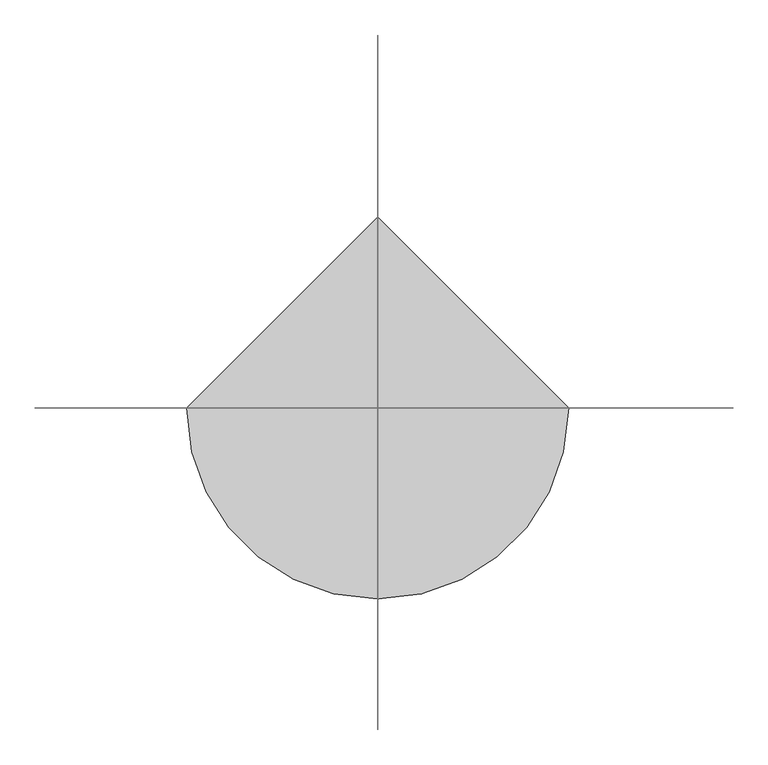
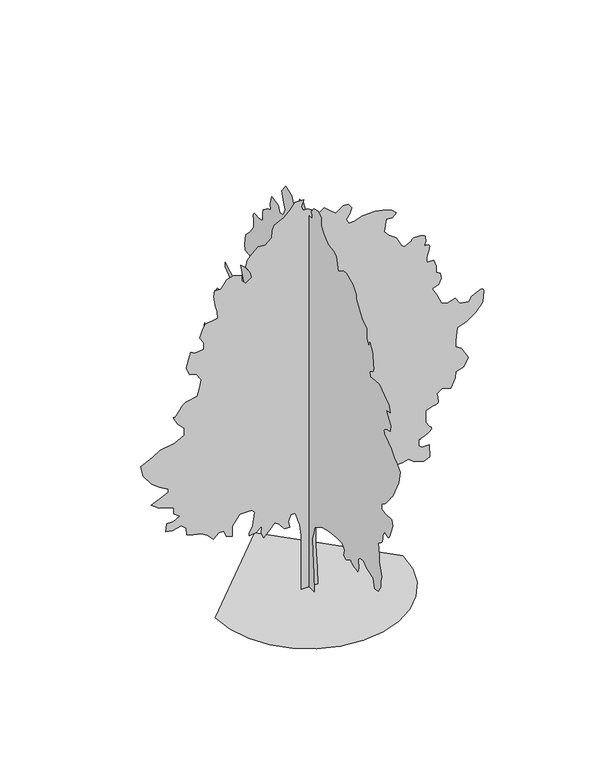
"""IFC4 building model written with IfcOpenShell, lengths in millimetres: geographic element geometry, RPC 木 - 落葉樹 : ベニカエデ - 9 メートル."""

from ifc_helpers import new_model, si_unit, origin, place, context, project, spatial, triangles, source, transform, mapped, element, save


def geographic_element_b7f9c851(model_context):
    return source(origin(), model_context, "Body", "Tessellation", [
        triangles([(5.8e-06, 197.3661507, 0.0129526), (5.8e-06, -197.3841547, 0.0129526), (5.8e-06, -171.0676287, 394.7628227), (5.8e-06, -144.750367, 907.9407286), (5.8e-06, -131.5926036, 1197.4234222), (5.8e-06, -171.0676287, 1342.1660408), (5.8e-06, -223.7014255, 1513.2237682), (5.8e-06, -315.8102654, 1565.8587822), (5.8e-06, -526.342909, 1684.2838211), (5.8e-06, -750.035614, 1736.9163643), (5.8e-06, -1052.6783329, 1776.3914257), (5.8e-06, -1263.2109764, 1776.3914257), (5.8e-06, -1355.318581, 1671.1238686), (5.8e-06, -1315.8435196, 1526.38125), (5.8e-06, -1421.1110767, 1486.9061886), (5.8e-06, -1592.1712749, 1579.016264), (5.8e-06, -1595.2388203, 1567.7362839), (5.8e-06, -1599.8038033, 1556.4587746), (5.8e-06, -1607.3613361, 1545.1812653), (5.8e-06, -1619.4088566, 1533.9012852), (5.8e-06, -1637.4388607, 1522.6237759), (5.8e-06, -1662.9487862, 1511.3436504), (5.8e-06, -1697.4363613, 1500.0661411), (5.8e-06, -1733.4588718, 1490.3212418), (5.8e-06, -1763.2689709, 1483.3386738), (5.8e-06, -1787.8963921, 1478.6611977), (5.8e-06, -1808.3814789, 1475.8211094), (5.8e-06, -1825.7589066, 1474.3636402), (5.8e-06, -1841.0664024, 1473.826173), (5.8e-06, -1855.3364616, 1473.7487068), (5.8e-06, -1881.6540413, 1565.8587822), (5.8e-06, -1868.4965595, 1763.2339439), (5.8e-06, -1947.446537, 1842.1839214), (5.8e-06, -2079.029203, 1855.3415485), (5.8e-06, -2184.2967602, 1750.0738461), (5.8e-06, -2434.3044651, 1671.1238686), (5.8e-06, -2500.1020477, 1473.7487068), (5.8e-06, -2618.5270866, 1486.9061886), (5.8e-06, -2723.7770576, 1644.8087597), (5.8e-06, -2723.7770576, 1776.3914257), (5.8e-06, -2750.102195, 1881.6589828), (5.8e-06, -2658.0020027, 2184.299231), (5.8e-06, -2658.0020027, 2355.3594292), (5.8e-06, -2631.6771561, 2618.5270866), (5.8e-06, -2634.7019714, 2618.6770775), (5.8e-06, -2639.0019997, 2619.7520119), (5.8e-06, -2645.8271645, 2622.677124), (5.8e-06, -2656.4520973, 2628.3520683), (5.8e-06, -2672.1520111, 2637.702079), (5.8e-06, -2694.1771202, 2651.6770981), (5.8e-06, -2723.7770576, 2671.1520721), (5.8e-06, -2752.6273315, 2695.2520546), (5.8e-06, -2772.5022812, 2722.1021599), (5.8e-06, -2784.9021057, 2751.2521248), (5.8e-06, -2791.3022964, 2782.2522675), (5.8e-06, -2793.227179, 2814.6273262), (5.8e-06, -2792.1522446, 2847.9273285), (5.8e-06, -2789.5771111, 2881.7023018), (5.8e-06, -2868.5272339, 3013.2774101), (5.8e-06, -2899.4523811, 2993.9524269), (5.8e-06, -2929.8022728, 2977.0272972), (5.8e-06, -2958.9772362, 2964.9524529), (5.8e-06, -2986.4523033, 2960.1024582), (5.8e-06, -3011.6275108, 2964.9524529), (5.8e-06, -3033.902314, 2981.8522934), (5.8e-06, -3052.7523262, 3013.2774101), (5.8e-06, -3184.3274345, 3329.0776108), (5.8e-06, -3144.8525185, 3460.6527191), (5.8e-06, -2894.8523712, 3447.5026497), (5.8e-06, -2750.102195, 3460.6527191), (5.8e-06, -2763.2522644, 3592.2528259), (5.8e-06, -2797.1272316, 3612.2277695), (5.8e-06, -2831.2521835, 3633.7029121), (5.8e-06, -2865.8024002, 3658.1778717), (5.8e-06, -2901.0522835, 3687.1528473), (5.8e-06, -2937.227401, 3722.1030396), (5.8e-06, -2974.5774467, 3764.5280663), (5.8e-06, -3013.2774101, 3815.9281265), (5.8e-06, -3049.3025368, 3866.5782326), (5.8e-06, -3079.102462, 3906.8530998), (5.8e-06, -3103.7274124, 3938.5032028), (5.8e-06, -3124.2276146, 3963.2531456), (5.8e-06, -3141.6024261, 3982.8031151), (5.8e-06, -3156.902655, 3998.9282936), (5.8e-06, -3171.1776558, 4013.3032883), (5.8e-06, -3394.8776642, 4460.7035957), (5.8e-06, -3460.6527191, 4750.1786591), (5.8e-06, -3315.9275414, 4908.0789047), (5.8e-06, -3250.1274879, 4921.2286835), (5.8e-06, -3105.3776024, 5105.4540665), (5.8e-06, -3013.2774101, 5171.2541199), (5.8e-06, -2976.8773064, 5188.2792435), (5.8e-06, -2941.9524033, 5206.0043243), (5.8e-06, -2910.027317, 5225.1043213), (5.8e-06, -2882.6022469, 5246.2791916), (5.8e-06, -2861.1773918, 5270.2294739), (5.8e-06, -2847.2023727, 5297.6039658), (5.8e-06, -2842.2023872, 5329.1543655), (5.8e-06, -2849.1272552, 5359.9042328), (5.8e-06, -2868.4522385, 5385.1544357), (5.8e-06, -2898.1524605, 5405.8043381), (5.8e-06, -2936.1274681, 5422.7544662), (5.8e-06, -2980.3273865, 5436.9541809), (5.8e-06, -3028.6523438, 5449.3045898), (5.8e-06, -3079.0524651, 5460.7294739), (5.8e-06, -3092.227533, 5605.4793594), (5.8e-06, -3026.4274796, 5710.7293304), (5.8e-06, -2921.1522194, 5855.4797974), (5.8e-06, -3079.0524651, 5894.9547134), (5.8e-06, -3026.4274796, 6052.8549591), (5.8e-06, -2855.3771645, 6158.1299286), (5.8e-06, -2658.0020027, 6302.8548157), (5.8e-06, -2486.9394791, 6289.7050369), (5.8e-06, -2329.0393787, 6276.5552582), (5.8e-06, -2302.7217991, 6381.8052292), (5.8e-06, -2381.6719219, 6434.4549225), (5.8e-06, -2395.6744102, 6437.4803192), (5.8e-06, -2409.1019337, 6441.7800568), (5.8e-06, -2421.3769112, 6448.6052216), (5.8e-06, -2431.9269939, 6459.2301544), (5.8e-06, -2440.1743103, 6474.9303589), (5.8e-06, -2445.5443314, 6496.9551773), (5.8e-06, -2447.464563, 6526.5551147), (5.8e-06, -2446.3120171, 6563.455188), (5.8e-06, -2443.0918648, 6605.8805054), (5.8e-06, -2438.1420216, 6652.9305405), (5.8e-06, -2431.8118847, 6703.6303528), (5.8e-06, -2424.4469273, 6757.1055771), (5.8e-06, -2416.3894249, 6812.4306885), (5.8e-06, -2407.9893562, 6868.6807434), (5.8e-06, -2302.7217991, 7052.905545), (5.8e-06, -2263.246883, 6947.6305756), (5.8e-06, -2197.4542419, 7066.0559052), (5.8e-06, -2197.4542419, 7316.0557617), (5.8e-06, -2026.3966599, 7421.3307312), (5.8e-06, -1907.9714756, 7579.2309769), (5.8e-06, -1789.5464367, 7750.2810013), (5.8e-06, -1789.5464367, 7842.406192), (5.8e-06, -1657.9612999, 8000.3064377), (5.8e-06, -1421.1110767, 8118.7317673), (5.8e-06, -1289.5285561, 8092.4066299), (5.8e-06, -1118.4684305, 7973.9813004), (5.8e-06, -1026.3608259, 8263.4566544), (5.8e-06, -934.2507505, 8329.2567078), (5.8e-06, -723.718107, 8355.5818451), (5.8e-06, -565.8179704, 8513.4820908), (5.8e-06, -460.552884, 8631.906839), (5.8e-06, -460.552884, 8816.1072235), (5.8e-06, -342.1277724, 8895.0570557), (5.8e-06, -184.2254012, 8855.5821396), (5.8e-06, -92.1178238, 8737.15681), (5.8e-06, -105.8898302, 8706.3569458), (5.8e-06, -117.7053427, 8676.8070053), (5.8e-06, -125.607849, 8649.8069092), (5.8e-06, -127.6411006, 8626.6071625), (5.8e-06, -121.8483492, 8608.4571075), (5.8e-06, -106.2730826, 8596.6316666), (5.8e-06, -78.9590612, 8592.4319229), (5.8e-06, 105.2585824, 8592.4319229), (5.8e-06, 223.6836758, 8763.4819473), (5.8e-06, 355.2677771, 8750.3321686), (5.8e-06, 421.0578383, 8592.4319229), (5.8e-06, 592.1179639, 8513.4820908), (5.8e-06, 657.9080252, 8645.0571991), (5.8e-06, 881.6006939, 8737.15681), (5.8e-06, 1026.3433125, 8539.7816483), (5.8e-06, 960.5507441, 8316.106929), (5.8e-06, 907.9182009, 8171.3564621), (5.8e-06, 973.7107693, 8013.4562164), (5.8e-06, 1105.2933626, 7987.1316605), (5.8e-06, 1157.9259058, 8131.881546), (5.8e-06, 1421.0936359, 8158.2066833), (5.8e-06, 1473.7286499, 7973.9813004), (5.8e-06, 1447.4112156, 7842.406192), (5.8e-06, 1565.8362545, 7802.9312759), (5.8e-06, 1736.8938366, 7671.3311691), (5.8e-06, 1750.0539345, 7579.2309769), (5.8e-06, 1750.0539345, 7421.3307312), (5.8e-06, 1815.8439594, 7381.8558151), (5.8e-06, 1973.7440598, 7381.8558151), (5.8e-06, 2004.5116585, 7387.106076), (5.8e-06, 2033.7816742, 7390.055896), (5.8e-06, 2060.05914, 7388.4059967), (5.8e-06, 2081.8492344, 7379.8559372), (5.8e-06, 2097.654229, 7362.1058578), (5.8e-06, 2105.9791569, 7332.8309006), (5.8e-06, 2105.3291965, 7289.7556229), (5.8e-06, 2100.4566742, 7242.4306046), (5.8e-06, 2096.9666256, 7201.3557861), (5.8e-06, 2094.6266521, 7165.4556519), (5.8e-06, 2093.2066807, 7133.6808472), (5.8e-06, 2092.476638, 7105.0308517), (5.8e-06, 2092.2092125, 7078.4307312), (5.8e-06, 2092.1717148, 7052.905545), (5.8e-06, 2223.7542355, 6868.6807434), (5.8e-06, 2394.8119629, 6697.6301376), (5.8e-06, 2434.286879, 6447.6052826), (5.8e-06, 2407.9719154, 6329.179953), (5.8e-06, 2276.3867786, 6316.0301743), (5.8e-06, 2171.1216923, 6289.7050369), (5.8e-06, 2092.1717148, 6118.6550125), (5.8e-06, 2197.4368011, 5921.2798508), (5.8e-06, 2434.286879, 5921.2798508), (5.8e-06, 2592.1769508, 5868.6295761), (5.8e-06, 2460.6044586, 5526.5295273), (5.8e-06, 2579.0271721, 5394.9294205), (5.8e-06, 2907.9774422, 5434.4043365), (5.8e-06, 3000.1023422, 5487.0546112), (5.8e-06, 3184.3024361, 5579.1542221), (5.8e-06, 3171.1526573, 5487.0546112), (5.8e-06, 2934.3022888, 5276.5040909), (5.8e-06, 2842.2023872, 4987.0287369), (5.8e-06, 2947.4523582, 4763.3287285), (5.8e-06, 3092.2025345, 4776.5037964), (5.8e-06, 3095.3773407, 4790.453817), (5.8e-06, 3100.752594, 4803.6288849), (5.8e-06, 3110.5025803, 4815.1787613), (5.8e-06, 3126.8024574, 4824.3037857), (5.8e-06, 3151.8523819, 4830.204007), (5.8e-06, 3187.8525101, 4832.0788925), (5.8e-06, 3236.9527107, 4829.1287819), (5.8e-06, 3473.8027885, 4802.8039352), (5.8e-06, 3592.2278275, 4631.7536201), (5.8e-06, 3552.7529114, 4447.5285278), (5.8e-06, 3408.0027351, 4342.2785568), (5.8e-06, 3289.5776962, 4052.7782043), (5.8e-06, 3342.2026817, 3868.5781105), (5.8e-06, 3394.8526657, 3802.7780571), (5.8e-06, 3526.427774, 3579.077758), (5.8e-06, 3789.6029892, 3605.4028954), (5.8e-06, 3960.6533043, 3710.6778648), (5.8e-06, 4013.2782898, 3473.827787), (5.8e-06, 3763.2781425, 3355.4027481), (5.8e-06, 3592.2278275, 3302.7527641), (5.8e-06, 3473.8027885, 3039.6025475), (5.8e-06, 3408.0027351, 2881.7023018), (5.8e-06, 3329.0526123, 2658.0020027), (5.8e-06, 3184.3024361, 2684.32714), (5.8e-06, 2960.6274261, 2723.8020561), (5.8e-06, 2776.4023338, 2684.32714), (5.8e-06, 2644.8272255, 2473.7844681), (5.8e-06, 2815.8772499, 2302.726886), (5.8e-06, 2973.7774956, 2276.4093063), (5.8e-06, 3000.1023422, 2026.3991306), (5.8e-06, 2988.6274612, 2001.2715946), (5.8e-06, 2976.0023598, 1977.6416416), (5.8e-06, 2961.0773987, 1957.0016224), (5.8e-06, 2942.7023575, 1940.8515907), (5.8e-06, 2919.7273064, 1930.6865135), (5.8e-06, 2891.0023155, 1928.001503), (5.8e-06, 2855.352166, 1934.291526), (5.8e-06, 2818.1771095, 1946.7215813), (5.8e-06, 2785.1520905, 1961.2215683), (5.8e-06, 2755.5771515, 1977.4490662), (5.8e-06, 2728.7520447, 1995.0590378), (5.8e-06, 2704.0271004, 2013.7016499), (5.8e-06, 2680.6520737, 2033.0366615), (5.8e-06, 2657.9770042, 2052.7167103), (5.8e-06, 2565.8771027, 2157.9842674), (5.8e-06, 2548.8019821, 2185.796814), (5.8e-06, 2530.801918, 2211.3067394), (5.8e-06, 2510.9769653, 2232.2143295), (5.8e-06, 2488.3795074, 2246.2168179), (5.8e-06, 2462.0994255, 2251.0117287), (5.8e-06, 2431.219479, 2244.2993477), (5.8e-06, 2394.8119629, 2223.7767632), (5.8e-06, 2349.1993401, 2197.1142918), (5.8e-06, 2292.5368103, 2173.2142971), (5.8e-06, 2226.6693192, 2151.6167782), (5.8e-06, 2153.4342545, 2131.8592632), (5.8e-06, 2074.6767071, 2113.484222), (5.8e-06, 1992.2365356, 2096.0291828), (5.8e-06, 1907.9540348, 2079.0341446), (5.8e-06, 1697.4189205, 2026.3991306), (5.8e-06, 1763.2114162, 1894.8164646), (5.8e-06, 1973.7440598, 1763.2339439), (5.8e-06, 2079.0116169, 1592.1737457), (5.8e-06, 1894.7940823, 1526.38125), (5.8e-06, 1869.3215092, 1526.5736801), (5.8e-06, 1843.2739712, 1527.9161854), (5.8e-06, 1816.0738873, 1531.5611664), (5.8e-06, 1787.1489086, 1538.6586983), (5.8e-06, 1755.9214542, 1550.3587109), (5.8e-06, 1721.8164139, 1567.8137501), (5.8e-06, 1684.2612934, 1592.1737457), (5.8e-06, 1645.5537724, 1620.7538326), (5.8e-06, 1608.2262543, 1650.0238483), (5.8e-06, 1572.0512821, 1679.8712997), (5.8e-06, 1536.7961666, 1710.1764267), (5.8e-06, 1502.2312706, 1740.8289162), (5.8e-06, 1468.1262302, 1771.7114788), (5.8e-06, 1434.2511177, 1802.7090054), (5.8e-06, 1171.085931, 1881.6589828), (5.8e-06, 960.5507441, 1921.1340443), (5.8e-06, 750.0181005, 1973.7665874), (5.8e-06, 539.4829136, 1934.291526), (5.8e-06, 249.9999474, 1829.0239689), (5.8e-06, 171.0498791, 1723.7588825), (5.8e-06, 105.2585824, 1539.5412025), (5.8e-06, 78.9410663, 1276.3735451), (5.8e-06, 105.2585824, 921.0982103), (5.8e-06, 157.8911256, 407.9228116), (-2052.3641155, 0.0, 0.0), (-1998.1065262, -470.2653726, 0.0), (-1843.5815105, -902.1306908, 0.0), (-1601.1612785, -1283.2184761, 0.0), (-1283.2184761, -1601.1612785, 0.0), (-902.1306908, -1843.5815105, 0.0), (-470.2653726, -1998.1065262, 0.0), (8.97e-05, -2052.3641155, 0.0), (470.2653726, -1998.1065262, 0.0), (902.1306908, -1843.5815105, 0.0), (1283.2184761, -1601.1612785, 0.0), (1601.1612785, -1283.2184761, 0.0), (1843.5815105, -902.1306908, 0.0), (1998.1065262, -470.2653726, 0.0), (2052.3641155, 0.0001799, 0.0), (-0.0002691, 2052.3641155, 0.0), (196.7396627, 0.0002249, 0.0051811), (-167.0323917, 0.0002249, 0.0051811), (-167.0323917, 0.0001889, 673.6580086), (-167.0323917, 0.0001619, 1023.9582836), (-167.0323917, 0.0001529, 1252.9985184), (-207.4516724, 0.0001349, 1508.988707), (-301.7627399, 0.0001169, 1805.3940159), (-396.0753153, 0.0001169, 1805.3940159), (-449.967847, 0.0001259, 1657.1912888), (-423.0203276, 0.0001349, 1522.4612858), (-544.2779334, 0.0001349, 1535.9337193), (-652.0630331, 0.0001259, 1670.6638676), (-746.3755903, 0.0001259, 1738.0289417), (-854.1581829, 0.0001259, 1616.7712269), (-988.8882586, 0.0001349, 1482.0412239), (-1042.7808266, 0.0001349, 1603.2987934), (-1029.3083204, 0.0001259, 1764.9764248), (-1164.0383961, 0.0001259, 1657.1912888), (-1312.243594, 0.0001259, 1643.7188553), (-1312.243594, 0.0001259, 1711.0839294), (-1231.4034702, 0.0001169, 1845.8139324), (-1190.9859518, 9.89e-05, 2142.2217121), (-1258.3509533, 9.89e-05, 2209.5867863), (-1514.3386711, 9.89e-05, 2209.5867863), (-1676.0138317, 0.0001079, 1980.5440807), (-1676.0138317, 0.0001169, 1886.2339943), (-1676.0138317, 0.0001259, 1751.503846), (-1810.7464508, 0.0001169, 1805.3940159), (-1864.6389462, 0.0001079, 1940.1264896), (-1972.4216114, 0.0001079, 1940.1264896), (-2093.6791809, 0.0001169, 1832.3414989), (-2228.4093292, 0.0001079, 1967.0715019), (-2363.1419483, 0.0001079, 2047.9091549), (-2538.3020416, 9.89e-05, 2088.3292168), (-2673.0272484, 9.89e-05, 2142.2217121), (-2686.5020073, 8.99e-05, 2290.4242939), (-2794.2771149, 8.1e-05, 2384.7368511), (-2996.3772789, 8.99e-05, 2344.3169346), (-3131.1024857, 8.1e-05, 2371.2644176), (-3117.6274361, 7.2e-05, 2546.4021286), (-2969.4274704, 7.2e-05, 2546.4021286), (-2834.7022636, 7.2e-05, 2627.2521355), (-2955.9524208, 6.3e-05, 2721.5521935), (-2955.9524208, 5.4e-05, 2856.3023987), (-3090.6773369, 5.4e-05, 2910.1773079), (-3279.302742, 5.4e-05, 2964.0775063), (-3454.4528069, 4.5e-05, 3098.8024223), (-3238.8775932, 3.6e-05, 3193.1274788), (-3077.202578, 3.6e-05, 3260.4777283), (-3077.202578, 2.7e-05, 3327.8526855), (-3279.302742, 1.8e-05, 3449.1028427), (-3440.9777573, 1.8e-05, 3570.3779984), (-3629.6028717, 0.0, 3826.3530716), (-3683.5030701, -1.8e-05, 4068.8783844), (-3575.7279625, -1.8e-05, 4122.7532936), (-3427.5027077, -2.7e-05, 4190.1282509), (-3252.3526428, -2.7e-05, 4297.9033585), (-2942.4773712, -3.6e-05, 4351.8035568), (-2726.9021576, -3.6e-05, 4459.5786644), (-2726.9021576, -4.5e-05, 4621.2536797), (-2875.1274124, -5.4e-05, 4769.4789345), (-2969.4274704, -7.2e-05, 4944.6289993), (-2960.6274261, -7.2e-05, 4942.0541565), (-2951.0024323, -7.2e-05, 4941.5041901), (-2939.7272484, -7.2e-05, 4944.978978), (-2925.9772156, -7.2e-05, 4954.4289825), (-2908.9273842, -7.2e-05, 4971.9040787), (-2887.7772217, -7.2e-05, 4999.4041443), (-2861.6523628, -7.2e-05, 5038.9290573), (-2833.9523094, -7.2e-05, 5080.8038269), (-2808.3771263, -8.1e-05, 5114.904071), (-2784.5771255, -8.1e-05, 5142.5041306), (-2762.17733, -8.1e-05, 5164.9289246), (-2740.8521782, -8.1e-05, 5183.4789551), (-2720.2272743, -8.1e-05, 5199.4291443), (-2699.9770569, -8.1e-05, 5214.0794128), (-2443.9793106, -8.99e-05, 5267.9790298), (-2390.0869606, -9.89e-05, 5456.6041443), (-2363.1419483, -0.0001079, 5618.2797409), (-2470.9270844, -0.0001169, 5779.9547562), (-2605.6520004, -0.0001169, 5820.3546158), (-2686.5020073, -0.0001349, 5995.5049713), (-2632.6020996, -0.0001439, 6184.1300858), (-2592.1769508, -0.0001529, 6332.3303421), (-2497.8719513, -0.0001439, 6278.4551422), (-2309.2493076, -0.0001529, 6305.4052414), (-2309.2493076, -0.0001619, 6453.6049164), (-2390.0869606, -0.0001619, 6588.3304138), (-2336.1943199, -0.0001709, 6736.5306702), (-2268.8292458, -0.0001799, 6871.2555862), (-1999.3690945, -0.0001889, 6911.6804443), (-2012.8416733, -0.0001979, 7073.3554596), (-2053.2615898, -0.0002069, 7221.5557159), (-2080.2066021, -0.0002159, 7437.1309296), (-2066.7341686, -0.0002249, 7571.8558456), (-1932.0040203, -0.0002249, 7558.3810867), (-1864.6389462, -0.0002249, 7639.2313843), (-1797.273872, -0.0002339, 7733.5314423), (-1662.5413982, -0.0002339, 7773.9563004), (-1473.9186092, -0.0002339, 7720.056102), (-1473.9186092, -0.0002249, 7598.8059448), (-1379.6086681, -0.0002249, 7504.5058868), (-1258.3509533, -0.0002249, 7598.8059448), (-1285.2959656, -0.0002339, 7733.5314423), (-1379.6086681, -0.0002429, 7881.7311172), (-1352.6610397, -0.0002519, 8029.9563721), (-1244.876049, -0.0002609, 8137.7317703), (-1110.1459007, -0.0002698, 8258.9813461), (-961.9432463, -0.0002609, 8245.5065872), (-813.7406645, -0.0002698, 8366.7817429), (-800.2656149, -0.0002788, 8514.9819992), (-759.8480965, -0.0002878, 8636.2321564), (-557.7504395, -0.0002968, 8730.5572128), (-436.4928337, -0.0002968, 8838.3320297), (-301.7627399, -0.0003058, 9000.007045), (-113.1403415, -0.0003058, 9000.007045), (-167.0323917, -0.0002968, 8851.80737), (-126.6133472, -0.0002968, 8757.4817322), (-32.3020254, -0.0002968, 8757.4817322), (48.5362907, -0.0002878, 8703.6071136), (75.4823112, -0.0002878, 8595.8067169), (237.1586891, -0.0002878, 8582.331958), (331.4702471, -0.0002878, 8649.7069153), (466.2003591, -0.0002788, 8541.9320984), (587.4579649, -0.0002788, 8434.1317017), (749.1355963, -0.0002788, 8555.4068573), (856.9206596, -0.0002788, 8555.4068573), (937.7582399, -0.0002788, 8447.6070419), (897.3382507, -0.0002698, 8312.8815445), (816.5006704, -0.0002609, 8218.5814865), (870.3931658, -0.0002609, 8110.7816711), (991.650808, -0.0002609, 8110.7816711), (1180.2734516, -0.0002609, 8178.1566284), (1449.7336029, -0.0002609, 8178.1566284), (1611.4112343, -0.0002609, 8151.2065292), (1813.5064568, -0.0002519, 8083.831572), (1907.819014, -0.0002519, 7989.531514), (1826.9788902, -0.0002429, 7895.2064575), (1692.2488873, -0.0002429, 7908.6812164), (1665.303875, -0.0002339, 7787.4310593), (1651.8288254, -0.0002249, 7639.2313843), (1746.1413826, -0.0002249, 7517.9812271), (1907.819014, -0.0002159, 7410.1808304), (2015.6016792, -0.0001979, 7194.6056168), (2082.966608, -0.0001979, 7140.7309982), (2244.6442394, -0.0002069, 7221.5557159), (2247.8267487, -0.0002069, 7233.0305969), (2252.7742664, -0.0002069, 7244.0305069), (2261.259359, -0.0002069, 7254.0810562), (2275.0468895, -0.0002069, 7262.7305283), (2295.9043373, -0.0002069, 7269.4806976), (2325.5993271, -0.0002069, 7273.8810104), (2365.9019543, -0.0002069, 7275.4559143), (2407.7743984, -0.0002069, 7273.8810104), (2441.8695557, -0.0002069, 7269.4806976), (2469.4844398, -0.0002069, 7262.7305283), (2491.91185, -0.0002069, 7254.0810562), (2510.4519974, -0.0002069, 7244.0305069), (2526.4018959, -0.0002069, 7233.0305969), (2541.0521645, -0.0002069, 7221.5557159), (2554.5269234, -0.0001979, 7100.3055588), (2527.5771149, -0.0001889, 7006.0055008), (2558.951944, -0.0001889, 7005.5555283), (2588.1021996, -0.0001889, 7002.5307129), (2612.7771469, -0.0001889, 6994.330632), (2630.7272141, -0.0001889, 6978.3304459), (2639.7272461, -0.0001889, 6951.9803101), (2637.5270897, -0.0001889, 6912.6553848), (2621.9021713, -0.0001799, 6857.780246), (2602.3272034, -0.0001799, 6799.7802979), (2589.127137, -0.0001799, 6751.6553284), (2581.2270378, -0.0001709, 6711.7804367), (2577.5769699, -0.0001709, 6678.5051422), (2577.1019989, -0.0001709, 6650.2051254), (2578.7521889, -0.0001709, 6625.1804901), (2581.4770226, -0.0001709, 6601.8051727), (2729.6772789, -0.0001709, 6601.8051727), (2783.5771866, -0.0001529, 6440.1301575), (2783.5771866, -0.0001529, 6305.4052414), (2877.8772446, -0.0001439, 6251.505043), (2891.3522942, -0.0001349, 6130.2548859), (2837.4523865, -0.0001349, 6008.9797302), (2702.7271797, -0.0001259, 5955.1045303), (2797.0522362, -0.0001169, 5779.9547562), (2891.3522942, -0.0001079, 5564.3795425), (3026.0775009, -9.89e-05, 5497.0045853), (3201.2275658, -0.0001079, 5550.9042023), (3295.5526222, -9.89e-05, 5402.7045273), (3497.6277878, -8.99e-05, 5375.7544281), (3565.0027451, -9.89e-05, 5470.0544861), (3619.4779083, -9.89e-05, 5501.3043228), (3671.7279167, -9.89e-05, 5529.3293564), (3719.5029076, -0.0001079, 5551.0291946), (3760.5280197, -0.0001079, 5563.1546173), (3792.6280952, -0.0001079, 5562.5796524), (3813.5279823, -0.0001079, 5546.0794968), (3821.0031075, -9.89e-05, 5510.4793442), (3820.2031563, -9.89e-05, 5465.8541611), (3818.0029999, -9.89e-05, 5424.0793854), (3814.6279152, -8.99e-05, 5384.6294678), (3810.3031792, -8.99e-05, 5347.0794342), (3805.2779045, -8.99e-05, 5310.9543137), (3799.7779495, -8.99e-05, 5275.7541367), (3794.0530083, -8.99e-05, 5241.0289307), (3645.8530426, -7.2e-05, 5079.3539154), (3457.2276375, -6.3e-05, 4931.1536591), (3241.6527145, -6.3e-05, 4863.7789925), (3214.7026154, -4.5e-05, 4567.3787704), (3214.7026154, -3.6e-05, 4432.6285652), (3335.9527725, -3.6e-05, 4351.8035568), (3484.1777367, -1.8e-05, 4095.8031944), (3389.8526802, -9e-06, 3907.2030785), (3214.7026154, 0.0, 3853.3031708), (3201.2275658, 9e-06, 3718.577964), (3106.9275078, 1.8e-05, 3503.0027504), (2918.3023933, 1.8e-05, 3570.3779984), (2801.5522522, 1.8e-05, 3481.1779198), (2800.6773056, 1.8e-05, 3482.6028328), (2800.3023285, 1.8e-05, 3481.8278801), (2800.9522888, 1.8e-05, 3476.6779037), (2803.1271561, 1.8e-05, 3464.9277489), (2807.3521889, 1.8e-05, 3444.4028389), (2814.1523552, 2.7e-05, 3412.9277252), (2823.9773369, 2.7e-05, 3368.2778343), (2830.0272583, 2.7e-05, 3322.9776924), (2826.1772026, 2.7e-05, 3289.7026886), (2814.0773598, 3.6e-05, 3266.4526543), (2795.4023369, 3.6e-05, 3251.202713), (2771.752327, 3.6e-05, 3241.9776947), (2744.8022278, 3.6e-05, 3236.7527229), (2716.2022293, 3.6e-05, 3233.5276291), (2554.5269234, 3.6e-05, 3179.6524292), (2554.5269234, 5.4e-05, 2910.1773079), (2635.3522224, 6.3e-05, 2788.9271507), (2655.0521828, 6.3e-05, 2771.5273407), (2671.5520477, 6.3e-05, 2753.652269), (2681.6770111, 6.3e-05, 2734.8272552), (2682.2522667, 6.3e-05, 2714.6020363), (2670.1271347, 6.3e-05, 2692.5022224), (2642.0771027, 7.2e-05, 2668.0272629), (2594.9520721, 7.2e-05, 2640.7271851), (2543.4770164, 7.2e-05, 2615.3769882), (2503.35214, 7.2e-05, 2596.4269821), (2472.6243645, 7.2e-05, 2582.7519447), (2449.4493256, 7.2e-05, 2573.3269386), (2431.9319355, 7.2e-05, 2567.0770294), (2418.1843735, 7.2e-05, 2562.9519905), (2406.3218708, 7.2e-05, 2559.8771782), (2406.3218708, 8.1e-05, 2425.156913), (2473.6870903, 8.99e-05, 2357.7893681), (2635.3522224, 8.99e-05, 2357.7893681), (2648.8269814, 9.89e-05, 2074.856638), (2514.1020653, 0.0001079, 2020.9641426), (2312.0093136, 9.89e-05, 2088.3292168), (2177.2793106, 9.89e-05, 2182.641774), (2042.5491623, 9.89e-05, 2155.6942909), (1800.0338779, 9.89e-05, 2142.2217121), (1651.8288254, 9.89e-05, 2101.8016502), (1638.3562466, 0.0001169, 1913.1790066), (1490.1536648, 0.0001169, 1899.7065731), (1301.5310211, 0.0001169, 1913.1790066), (1220.6910427, 0.0001169, 1791.9214371), (937.7582399, 0.0001259, 1751.503846), (722.1881132, 0.0001169, 1805.3940159), (722.1881132, 0.0001349, 1589.8262146), (547.0404465, 0.0001349, 1603.2987934), (493.1478785, 0.0001259, 1711.0839294), (398.8353212, 0.0001259, 1670.6638676), (291.0502397, 0.0001259, 1670.6638676), (250.6327031, 0.0001169, 1791.9214371), (142.8473672, 0.0001259, 1670.6638676), (129.3743524, 0.0001349, 1522.4612858), (142.8473672, 0.0001529, 1293.4185802), (142.8473672, 0.0001709, 916.1732203), (183.2666479, 0.0002069, 377.2503016)], [[130, 131, 132], [208, 209, 210], [208, 210, 211], [207, 208, 211], [230, 231, 232], [230, 232, 233], [276, 277, 278], [229, 230, 233], [229, 233, 234], [302, 1, 2], [302, 2, 3], [302, 3, 4], [301, 302, 4], [301, 4, 5], [300, 301, 5], [300, 5, 6], [299, 300, 6], [299, 6, 7], [108, 109, 110], [203, 204, 205], [206, 207, 211], [206, 211, 212], [108, 110, 111], [202, 203, 205], [13, 14, 15], [13, 15, 16], [236, 237, 238], [171, 172, 173], [170, 171, 173], [170, 173, 174], [36, 37, 38], [36, 38, 39], [36, 39, 40], [275, 276, 278], [275, 278, 279], [275, 279, 280], [275, 280, 281], [275, 281, 282], [275, 282, 283], [275, 283, 284], [275, 284, 285], [275, 285, 286], [275, 286, 287], [275, 287, 288], [275, 288, 289], [275, 289, 290], [274, 275, 290], [274, 290, 291], [274, 291, 292], [67, 68, 69], [66, 67, 69], [164, 165, 166], [164, 166, 167], [163, 164, 167], [163, 167, 168], [242, 243, 244], [29, 30, 31], [104, 105, 106], [197, 198, 199], [28, 29, 31], [298, 299, 7], [66, 69, 70], [65, 66, 70], [64, 65, 70], [63, 64, 70], [62, 63, 70], [61, 62, 70], [60, 61, 70], [59, 60, 70], [27, 28, 31], [150, 151, 152], [160, 161, 162], [159, 160, 162], [196, 197, 199], [195, 196, 199], [195, 199, 200], [26, 27, 31], [133, 134, 135], [242, 244, 245], [242, 245, 246], [242, 246, 247], [242, 247, 248], [242, 248, 249], [242, 249, 250], [242, 250, 251], [242, 251, 252], [242, 252, 253], [242, 253, 254], [242, 254, 255], [242, 255, 256], [242, 256, 257], [242, 257, 258], [242, 258, 259], [241, 242, 259], [241, 259, 260], [241, 260, 261], [241, 261, 262], [241, 262, 263], [241, 263, 264], [298, 7, 8], [274, 292, 293], [147, 148, 149], [147, 149, 150], [147, 150, 152], [147, 152, 153], [147, 153, 154], [147, 154, 155], [147, 155, 156], [36, 40, 41], [36, 41, 42], [35, 36, 42], [34, 35, 42], [34, 42, 43], [86, 87, 88], [86, 88, 89], [34, 43, 44], [104, 106, 107], [103, 104, 107], [102, 103, 107], [25, 26, 31], [25, 31, 32], [24, 25, 32], [23, 24, 32], [22, 23, 32], [21, 22, 32], [20, 21, 32], [19, 20, 32], [18, 19, 32], [17, 18, 32], [16, 17, 32], [13, 16, 32], [12, 13, 32], [102, 107, 108], [101, 102, 108], [129, 130, 132], [146, 147, 156], [100, 101, 108], [236, 238, 239], [146, 156, 157], [221, 222, 223], [221, 223, 224], [221, 224, 225], [220, 221, 225], [219, 220, 225], [218, 219, 225], [217, 218, 225], [216, 217, 225], [215, 216, 225], [214, 215, 225], [213, 214, 225], [213, 225, 226], [33, 34, 44], [235, 236, 239], [298, 8, 9], [297, 298, 9], [12, 32, 33], [58, 59, 70], [175, 176, 177], [85, 86, 89], [85, 89, 90], [85, 90, 91], [85, 91, 92], [84, 85, 92], [84, 92, 93], [83, 84, 93], [82, 83, 93], [82, 93, 94], [81, 82, 94], [80, 81, 94], [80, 94, 95], [79, 80, 95], [12, 33, 44], [78, 79, 95], [77, 78, 95], [76, 77, 95], [75, 76, 95], [74, 75, 95], [73, 74, 95], [72, 73, 95], [71, 72, 95], [71, 95, 96], [108, 111, 112], [108, 112, 113], [100, 108, 113], [100, 113, 114], [99, 100, 114], [98, 99, 114], [194, 195, 200], [128, 129, 132], [137, 138, 139], [175, 177, 178], [174, 175, 178], [241, 264, 265], [139, 140, 141], [139, 141, 142], [137, 139, 142], [229, 234, 235], [229, 235, 239], [228, 229, 239], [227, 228, 239], [227, 239, 240], [226, 227, 240], [213, 226, 240], [136, 137, 142], [142, 143, 144], [142, 144, 145], [145, 146, 157], [127, 128, 132], [11, 12, 44], [170, 174, 178], [194, 200, 201], [71, 96, 97], [145, 157, 158], [169, 170, 178], [212, 213, 240], [206, 212, 240], [205, 206, 240], [205, 240, 241], [205, 241, 265], [205, 265, 266], [205, 266, 267], [205, 267, 268], [205, 268, 269], [205, 269, 270], [205, 270, 271], [205, 271, 272], [205, 272, 273], [205, 273, 274], [205, 274, 293], [205, 293, 294], [205, 294, 295], [202, 205, 295], [202, 295, 296], [201, 202, 296], [201, 296, 297], [201, 297, 9], [201, 9, 10], [201, 10, 11], [201, 11, 44], [194, 201, 44], [193, 194, 44], [193, 44, 45], [193, 45, 46], [193, 46, 47], [193, 47, 48], [193, 48, 49], [193, 49, 50], [193, 50, 51], [193, 51, 52], [193, 52, 53], [193, 53, 54], [193, 54, 55], [193, 55, 56], [193, 56, 57], [193, 57, 58], [193, 58, 70], [193, 70, 71], [193, 71, 97], [193, 97, 98], [193, 98, 114], [193, 114, 115], [192, 193, 115], [191, 192, 115], [190, 191, 115], [189, 190, 115], [188, 189, 115], [187, 188, 115], [186, 187, 115], [185, 186, 115], [184, 185, 115], [183, 184, 115], [182, 183, 115], [181, 182, 115], [180, 181, 115], [179, 180, 115], [178, 179, 115], [169, 178, 115], [168, 169, 115], [163, 168, 115], [162, 163, 115], [159, 162, 115], [158, 159, 115], [145, 158, 115], [142, 145, 115], [136, 142, 115], [135, 136, 115], [133, 135, 115], [132, 133, 115], [127, 132, 115], [126, 127, 115], [126, 115, 116], [125, 126, 116], [124, 125, 116], [123, 124, 116], [122, 123, 116], [121, 122, 116], [121, 116, 117], [120, 121, 117], [120, 117, 118], [119, 120, 118], [317, 318, 303], [316, 317, 303], [316, 303, 304], [315, 316, 304], [315, 304, 305], [315, 305, 306], [314, 315, 306], [313, 314, 306], [313, 306, 307], [313, 307, 308], [313, 308, 309], [313, 309, 310], [313, 310, 311], [313, 311, 312], [379, 380, 381], [379, 381, 382], [364, 365, 366], [344, 345, 346], [332, 333, 334], [433, 434, 435], [327, 328, 329], [401, 402, 403], [327, 329, 330], [344, 346, 347], [343, 344, 347], [332, 334, 335], [432, 433, 435], [379, 382, 383], [534, 535, 536], [336, 337, 338], [336, 338, 339], [335, 336, 339], [582, 583, 584], [582, 584, 585], [593, 319, 320], [593, 320, 321], [592, 593, 321], [592, 321, 322], [591, 592, 322], [591, 322, 323], [412, 413, 414], [331, 332, 335], [591, 323, 324], [590, 591, 324], [568, 569, 570], [568, 570, 571], [568, 571, 572], [568, 572, 573], [567, 568, 573], [348, 349, 350], [532, 533, 534], [454, 455, 456], [454, 456, 457], [453, 454, 457], [357, 358, 359], [356, 357, 359], [355, 356, 359], [355, 359, 360], [363, 364, 366], [363, 366, 367], [589, 590, 324], [589, 324, 325], [576, 577, 578], [371, 372, 373], [335, 339, 340], [379, 383, 384], [504, 505, 506], [440, 441, 442], [417, 418, 419], [326, 327, 330], [494, 495, 496], [586, 587, 588], [362, 363, 367], [432, 435, 436], [588, 589, 325], [326, 330, 331], [352, 353, 354], [585, 586, 588], [452, 453, 457], [331, 335, 340], [379, 384, 385], [416, 417, 419], [415, 416, 419], [411, 412, 414], [531, 532, 534], [528, 529, 530], [528, 530, 531], [527, 528, 531], [431, 432, 436], [414, 415, 419], [411, 414, 419], [411, 419, 420], [410, 411, 420], [409, 410, 420], [576, 578, 579], [371, 373, 374], [370, 371, 374], [370, 374, 375], [369, 370, 375], [369, 375, 376], [368, 369, 376], [368, 376, 377], [407, 408, 409], [452, 457, 458], [451, 452, 458], [450, 451, 458], [450, 458, 459], [497, 498, 499], [497, 499, 500], [497, 500, 501], [445, 446, 447], [444, 445, 447], [443, 444, 447], [443, 447, 448], [326, 331, 340], [360, 361, 362], [494, 496, 497], [405, 406, 407], [405, 407, 409], [398, 399, 400], [398, 400, 401], [398, 401, 403], [398, 403, 404], [397, 398, 404], [579, 580, 581], [494, 497, 501], [425, 426, 427], [379, 385, 386], [429, 430, 431], [527, 531, 534], [477, 478, 479], [476, 477, 479], [475, 476, 479], [474, 475, 479], [473, 474, 479], [473, 479, 480], [472, 473, 480], [471, 472, 480], [470, 471, 480], [469, 470, 480], [468, 469, 480], [467, 468, 480], [466, 467, 480], [465, 466, 480], [464, 465, 480], [463, 464, 480], [566, 567, 573], [566, 573, 574], [566, 574, 575], [428, 429, 431], [428, 431, 436], [422, 423, 424], [422, 424, 425], [422, 425, 427], [421, 422, 427], [342, 343, 347], [437, 438, 439], [436, 437, 439], [428, 436, 439], [378, 379, 386], [378, 386, 387], [378, 387, 388], [378, 388, 389], [378, 389, 390], [378, 390, 391], [378, 391, 392], [378, 392, 393], [378, 393, 394], [378, 394, 395], [582, 585, 588], [351, 352, 354], [513, 514, 515], [512, 513, 515], [511, 512, 515], [511, 515, 516], [510, 511, 516], [510, 516, 517], [509, 510, 517], [509, 517, 518], [509, 518, 519], [508, 509, 519], [507, 508, 519], [507, 519, 520], [507, 520, 521], [507, 521, 522], [507, 522, 523], [507, 523, 524], [506, 507, 524], [506, 524, 525], [504, 506, 525], [503, 504, 525], [354, 355, 360], [579, 581, 582], [342, 347, 348], [342, 348, 350], [342, 350, 351], [342, 351, 354], [342, 354, 360], [342, 360, 362], [342, 362, 367], [342, 367, 368], [342, 368, 377], [341, 342, 377], [449, 450, 459], [527, 534, 536], [404, 405, 409], [341, 377, 378], [341, 378, 395], [341, 395, 396], [503, 525, 526], [440, 442, 443], [555, 556, 557], [554, 555, 557], [554, 557, 558], [553, 554, 558], [552, 553, 558], [552, 558, 559], [551, 552, 559], [551, 559, 560], [551, 560, 561], [551, 561, 562], [551, 562, 563], [551, 563, 564], [551, 564, 565], [551, 565, 566], [551, 566, 575], [550, 551, 575], [550, 575, 576], [460, 461, 462], [483, 484, 485], [482, 483, 485], [482, 485, 486], [481, 482, 486], [481, 486, 487], [480, 481, 487], [480, 487, 488], [463, 480, 488], [463, 488, 489], [463, 489, 490], [463, 490, 491], [463, 491, 492], [463, 492, 493], [463, 493, 494], [463, 494, 501], [341, 396, 397], [340, 341, 397], [326, 340, 397], [325, 326, 397], [588, 325, 397], [582, 588, 397], [579, 582, 397], [576, 579, 397], [550, 576, 397], [550, 397, 404], [550, 404, 409], [550, 409, 420], [550, 420, 421], [549, 550, 421], [549, 421, 427], [549, 427, 428], [549, 428, 439], [549, 439, 440], [549, 440, 443], [549, 443, 448], [549, 448, 449], [549, 449, 459], [549, 459, 460], [549, 460, 462], [549, 462, 463], [549, 463, 501], [549, 501, 502], [549, 502, 503], [548, 549, 503], [547, 548, 503], [526, 527, 536], [503, 526, 536], [544, 545, 546], [543, 544, 546], [543, 546, 547], [542, 543, 547], [541, 542, 547], [540, 541, 547], [503, 536, 537], [547, 503, 537], [547, 537, 538], [547, 538, 539], [540, 547, 539]], closed=False),
    ])


if __name__ == "__main__":
    model = new_model("IFC4")
    model_context = context("Model", 3, world=origin())
    ifc_project = project(units=[si_unit("LENGTHUNIT", "METRE", prefix="MILLI")], contexts=[model_context])
    site = spatial("IfcSite", under=ifc_project)
    building = spatial("IfcBuilding", under=site)
    placement = place(None, origin())
    geographic_element_shape = geographic_element_b7f9c851(model_context)
    element("IfcGeographicElement", 1, ObjectType="RPC 木 - 落葉樹 : ベニカエデ - 9 メートル", at=placement, inside=building, context=model_context, shape_type="MappedRepresentation", body=[
        mapped(geographic_element_shape, transform((0.0, 0.0, 0.0), x_axis=(1.0, 0.0, 0.0), y_axis=(0.0, 1.0, 0.0), z_axis=(0.0, 0.0, 1.0))),
    ])
    save(model, "model.ifc")

# Revit data of these elements
# Type "RPC 木 - 落葉樹 : ベニカエデ - 9 メートル"
#   built-in parameter 1005198 = "{2, 15},{39, RPC-16-G0SR-83PX-Q347-6000-ST1L-LVER-AU},{1, 0},{1, 0},{2, 35},{1, 8},{5, Color},{1, 0},{1, 0},{3, 0.8},{3, 0.8},{3, 0.8},{1, 8},{7, BBoxMin},{1, 0},{1, 0},{1, 0},{1, 0},{1, 0},{1, 8},{7, BBoxMax},{1, 0},{1, 0},{1, 0},{1, 0},{1, 0},{2, 11},{9, RPCTypeId},{1, 0},{1, 0},{39, RPC-16-G0SR-83PX-Q347-6000-ST1L-LVER-AU},{1, 6},{14, RPCPlantHeight},{1, 0},{1, 0},{7, 29.5276},{2, 11},{7, keyword},{1, 0},{1, 0},{241, :Geometry:RPC:Red Maple:A common species of the forests of eastern North America:ranging as far south as Florida.  Widely planted as a shade tree.  The twings:buds:flowers:immature fruits:leaf stalks:and autumn leaves are usually bright red.},{2, 11},{8, category},{1, 0},{1, 0},{16, :Trees [General]},{2, 11},{12, LocalizedUID},{1, 0},{1, 0},{9, Red Maple},{2, 14},{6, Height},{1, 0},{1, 0},{7, 29.5276},{1, 2},{16, Cast Reflections},{1, 0},{1, 0},{1, 0},{1, 2},{12, Cast Shadows},{1, 0},{1, 0},{1, 1},{1, 2},{9, Lock View},{1, 0},{1, 0},{1, 0},{1, 4},{5, ViewC},{1, 0},{1, 0},{1, 0},{2, 11},{20, AdvancedUIDefinition},{1, 0},{1, 0},{0, },{2, 11},{10, AssetLibID},{1, 0},{1, 0},{36, 4D3F6E72-3F99-4203-98E9-AF80B3C7A7A4},{2, 11},{10, BaseSchema},{1, 0},{1, 0},{9, RPCSchema},{2, 11},{12, ExchangeGUID},{1, 0},{1, 0},{0, },{1, 2},{6, Hidden},{1, 0},{1, 0},{1, 0},{1, 4},{11, RPCCategory},{1, 0},{1, 0},{1, 0},{2, 11},{8, RPCImage},{1, 0},{1, 0},{0, },{1, 4},{13, SchemaVersion},{1, 0},{1, 0},{1, 4},{2, 11},{12, UIDefinition},{1, 0},{1, 0},{0, },{2, 11},{6, UIName},{1, 0},{1, 0},{39, RPC-16-G0SR-83PX-Q347-6000-ST1L-LVER-AU},{2, 11},{11, VersionGUID},{1, 0},{1, 0},{9, RPCSchema},{2, 11},{9, assettype},{1, 0},{1, 0},{11, RPCGeometry},{2, 11},{11, description},{1, 0},{1, 0},{0, },{2, 11},{9, localname},{1, 0},{1, 0},{3, RPC},{2, 11},{9, localtype},{1, 0},{1, 0},{3, RPC},{1, 4},{8, revision},{1, 0},{1, 0},{1, 1},{2, 11},{9, thumbnail},{1, 0},{1, 0},{0, },{1, 4},{7, version},{1, 0},{1, 0},{1, 1},{1, 2},{20, RPC_Cast Reflections},{1, 0},{1, 0},{1, 1},{1, 2},{16, RPC_Cast Shadows},{1, 0},{1, 0},{1, 1},{1, 2},{13, RPC_Lock View},{1, 0},{1, 0},{1, 0},{1, 4},{9, RPC_ViewC},{1, 0},{1, 0},{1, 0},{21, assetlibrary_base.fbx},{1, 5},"
#   built-in parameter 1005195 = "RPC-16-G0SR-83PX-Q347-6000-ST1L-LVER-AU"
#   Type Comments = "赤カエデ"
#   Height = 9000 mm
#   Default Elevation = 0
